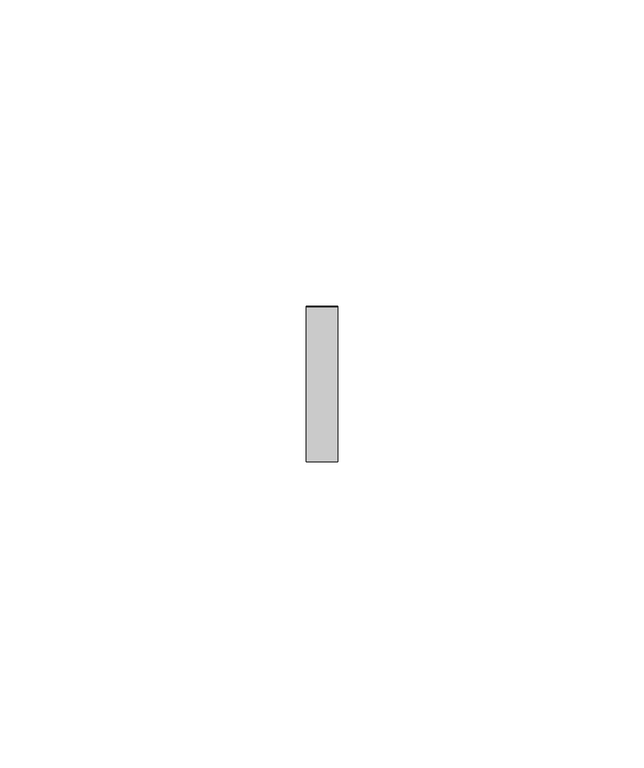
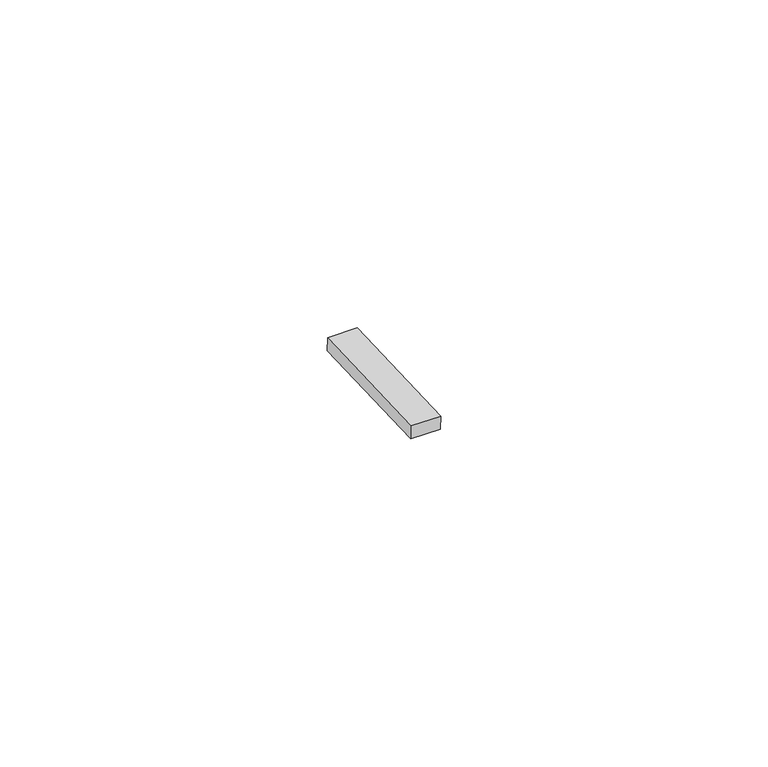
"""IFC4 building model written with IfcOpenShell, lengths in millimetres: proxy geometry, Inner panel:Inner panel:1:Inner panel:1 : Inner panel:Inner panel:300324:2:Inner panel:1:Inner panel:1 : Inner panel:Inner panel:300324:2 : Inner panel:Inner panel:1:Inner panel:1 : Inner panel:Inner panel:300324:300043:93 : Inner panel:Inner panel:1:Inner panel:1 : Inner panel:Inner panel:300324:2:Inner panel:1:Inner panel:1 : Inner panel:Inner panel:300324:2 : Inner panel:Inner panel:1:Inner panel:1 : Inner panel:Inner panel:300324:300043:308120."""

from ifc_helpers import new_model, si_unit, frame, origin, place, context, project, spatial, polyline, outline, extrude, source, transform, mapped, element, save


def generic_models_218dd8f9(model_context):
    return source(origin(), model_context, "Body", "SweptSolid", [
        extrude(outline(polyline([(0.0, -25.3999999), (0.0, 0.0), (5.2138089, 0.0), (5.2138089, -25.3999999), (0.0, -25.3999999)])), frame((591904.595117, -566905.6162814, 8857.0720004), z_axis=(0.0, -0.041630544712223896, 0.9991330730923502), x_axis=(-1.0, 0.0, 0.0)), (0.0, 0.0, 1.0), 2.4763745),
    ])


if __name__ == "__main__":
    model = new_model("IFC4")
    model_context = context("Model", 3, world=origin())
    ifc_project = project(units=[si_unit("LENGTHUNIT", "METRE", prefix="MILLI")], contexts=[model_context])
    site = spatial("IfcSite", under=ifc_project)
    building = spatial("IfcBuilding", under=site)
    placement = place(None, origin())
    generic_models_shape = generic_models_218dd8f9(model_context)
    element("IfcBuildingElementProxy", 1, Name="Inner panel:Inner panel:1:Inner panel:1 : Inner panel:Inner panel:300324:2:Inner panel:1:Inner panel:1 : Inner panel:Inner panel:300324:2 : Inner panel:Inner panel:1:Inner panel:1 : Inner panel:Inner panel:300324:300043:93 : Inner panel:Inner panel:1:Inner panel:1 : Inner panel:Inner panel:300324:2:Inner panel:1:Inner panel:1 : Inner panel:Inner panel:300324:2 : Inner panel:Inner panel:1:Inner panel:1 : Inner panel:Inner panel:300324:300043:308120", ObjectType="Inner panel:Inner panel:1:Inner panel:1 : Inner panel:Inner panel:300324:2:Inner panel:1:Inner panel:1 : Inner panel:Inner panel:300324:2 : Inner panel:Inner panel:1:Inner panel:1 : Inner panel:Inner panel:300324:300043:93 : Inner panel:Inner panel:1:Inner panel:1 : Inner panel:Inner panel:300324:2:Inner panel:1:Inner panel:1 : Inner panel:Inner panel:300324:2 : Inner panel:Inner panel:1:Inner panel:1 : Inner panel:Inner panel:300324:300043:308120", at=placement, inside=building, context=model_context, shape_type="MappedRepresentation", body=[
        mapped(generic_models_shape, transform((0.0, 0.0, 0.0), x_axis=(1.0, 0.0, 0.0), y_axis=(0.0, 1.0, 0.0), z_axis=(0.0, 0.0, 1.0))),
    ])
    save(model, "model.ifc")

# Revit data of these elements
# Type "Inner panel:Inner panel:1:Inner panel:1 : Inner panel:Inner panel:300324:2:Inner panel:1:Inner panel:1 : Inner panel:Inner panel:300324:2 : Inner panel:Inner panel:1:Inner panel:1 : Inner panel:Inner panel:300324:300043:93 : Inner panel:Inner panel:1:Inner panel:1 : Inner panel:Inner panel:300324:2:Inner panel:1:Inner panel:1 : Inner panel:Inner panel:300324:2 : Inner panel:Inner panel:1:Inner panel:1 : Inner panel:Inner panel:300324:300043:308120"
#   NameOverride = "Inner panel:Inner panel:1:Inner panel:1 : Inner panel:Inner panel:300324:2:Inner panel:1:Inner panel:1 : Inner panel:Inner panel:300324:2 : Inner panel:Inner panel:1:Inner panel:1 : Inner panel:Inner panel:300324:300043:308120"
#   ObjectTypeOverride = "Inner panel:1:Inner panel:1 : Inner panel:Inner panel:300324:2 : Inner panel:Inner panel:1:Inner panel:1 : Inner panel:Inner panel:300324:300043"
#   Reference = "Inner panel"
#   Tag = "308120"
# Element 1 (IfcBuildingElementProxy, "Inner panel:Inner panel:1:Inner panel:1 : Inner panel:Inner panel:300324:2:Inner panel:1:Inner panel:1 : Inner panel:Inner panel:300324:2 : Inner panel:Inner panel:1:Inner panel:1 : Inner panel:Inner panel:300324:300043:93 : Inner panel:Inner panel:1:Inner panel:1 : Inner panel:Inner panel:300324:2:Inner panel:1:Inner panel:1 : Inner panel:Inner panel:300324:2 : Inner panel:Inner panel:1:Inner panel:1 : Inner panel:Inner panel:300324:300043:308120")
#   Materials on its faces: "AT CLIP - 1\" WIDE NON ABSORBENT, WEATHER-RESISTANT NEOPRENE/EPDM/SBR FOAM"
# Materials
#   "AT CLIP - 1\" WIDE NON ABSORBENT, WEATHER-RESISTANT NEOPRENE/EPDM/SBR FOAM": class "Generic", colour RGB 85 85 85, transparency 0, Cost = 0
